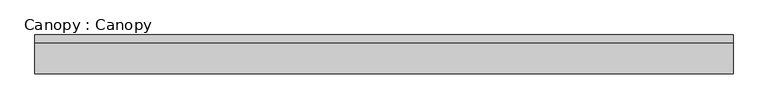
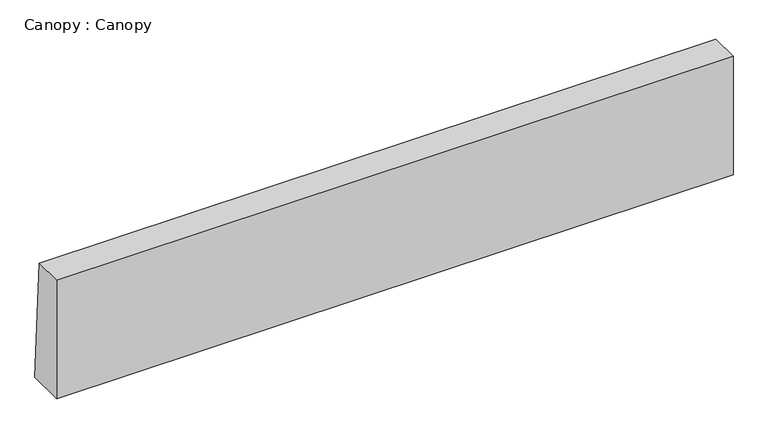
"""IFC4 building model written with IfcOpenShell, lengths in millimetres: proxy geometry, Canopy : Canopy."""

import ifcopenshell
import ifcopenshell.guid

model = None  # the IFC model being written
_history = None  # IfcOwnerHistory: only IFC2X3 demands one
_inside = {}  # id of a spatial element -> (the spatial element, [elements in it])
_under = {}  # id of a project, library or spatial element -> (it, [spatial elements below it])
_declared = {}  # id of a project -> (the project, [libraries it declares])
_typed = {}  # id of a type object -> (the type object, [elements of that type])
_made_of = {}  # id of a material, layer set ... -> (it, [elements and type objects made of it])


def new_model(schema):
    """Start an empty IFC model of exactly this schema.

    Asked for "IFC4X3", IfcOpenShell would pick the latest addendum, in which some entities
    have other attributes; the version numbers below select the first issue.
    IFC2X3 requires an IfcOwnerHistory on every rooted entity: one is made here for all.
    """
    global model, _history
    if schema == "IFC4X3":
        model = ifcopenshell.file(schema_version=(4, 3, 0, 0))
    else:
        model = ifcopenshell.file(schema=schema)
    _inside.clear()
    _under.clear()
    _declared.clear()
    _typed.clear()
    _made_of.clear()
    _history = None
    if model.schema == "IFC2X3":
        org = make("IfcOrganization", Name="unknown")
        user = make(
            "IfcPersonAndOrganization",
            ThePerson=make("IfcPerson", FamilyName="unknown"),
            TheOrganization=org,
        )
        app = make(
            "IfcApplication",
            ApplicationDeveloper=org,
            Version="unknown",
            ApplicationFullName="unknown",
            ApplicationIdentifier="unknown",
        )
        _history = make(
            "IfcOwnerHistory",
            OwningUser=user,
            OwningApplication=app,
            ChangeAction="ADDED",
            CreationDate=0,
        )
    return model


def make(cls, **values):
    """One entity of the class cls with the attributes given. An attribute that is None is left unset."""
    return model.create_entity(
        cls, **{name: value for name, value in values.items() if value is not None}
    )


def rooted(cls, **values):
    """An entity with a GlobalId (a new one), such as an element, a storey or a relation."""
    return make(cls, GlobalId=ifcopenshell.guid.new(), OwnerHistory=_history, **values)


def si_unit(unit_type, name, prefix=None):
    """IfcSIUnit, for example si_unit("LENGTHUNIT", "METRE", prefix="MILLI")."""
    return make("IfcSIUnit", UnitType=unit_type, Prefix=prefix, Name=name)


def assignment(units):
    """IfcUnitAssignment: the units of a project."""
    return None if units is None else make("IfcUnitAssignment", Units=units)


def point(xyz):
    """IfcCartesianPoint."""
    return None if xyz is None else make("IfcCartesianPoint", Coordinates=xyz)


def direction(xyz):
    """IfcDirection."""
    return None if xyz is None else make("IfcDirection", DirectionRatios=xyz)


def frame(location, z_axis=None, x_axis=None):
    """IfcAxis2Placement3D, a coordinate frame: its origin and axes. An axis left out is left unset."""
    return make(
        "IfcAxis2Placement3D",
        Location=point(location),
        Axis=direction(z_axis),
        RefDirection=direction(x_axis),
    )


def origin():
    """The frame at (0, 0, 0) with its axes left unset."""
    return frame((0.0, 0.0, 0.0))


def place(relative_to, where):
    """IfcLocalPlacement: puts the frame where relative to a parent placement (None: the world)."""
    return make(
        "IfcLocalPlacement", PlacementRelTo=relative_to, RelativePlacement=where
    )


def context(
    kind, dimensions, precision=None, world=None, true_north=None, identifier=None
):
    """IfcGeometricRepresentationContext, for example the 3D "Model" context."""
    return make(
        "IfcGeometricRepresentationContext",
        ContextIdentifier=identifier,
        ContextType=kind,
        CoordinateSpaceDimension=dimensions,
        Precision=precision,
        WorldCoordinateSystem=world,
        TrueNorth=true_north,
    )


def project(units=None, contexts=None):
    """IfcProject with its units and contexts."""
    return rooted(
        "IfcProject",
        Name="project",
        RepresentationContexts=contexts,
        UnitsInContext=assignment(units),
    )


def spatial(cls, under=None, at=None, **own):
    """A site, building, storey or space (cls), placed at a placement, below another one or the project."""
    s = rooted(cls, ObjectPlacement=at, **own)
    if under is not None:
        _under.setdefault(under.id(), (under, []))[1].append(s)
    return s


def polyline(points):
    """IfcPolyline through the points."""
    return make("IfcPolyline", Points=[point(p) for p in points])


def outline(outer, holes=None, kind="AREA"):
    """IfcArbitraryClosedProfileDef: a profile drawn as a closed curve; with holes, ...WithVoids."""
    if holes is None:
        return make("IfcArbitraryClosedProfileDef", ProfileType=kind, OuterCurve=outer)
    return make(
        "IfcArbitraryProfileDefWithVoids",
        ProfileType=kind,
        OuterCurve=outer,
        InnerCurves=holes,
    )


def extrude(swept, where, along, depth):
    """IfcExtrudedAreaSolid: the profile swept, set in the frame where, extruded along a direction by depth."""
    return make(
        "IfcExtrudedAreaSolid",
        SweptArea=swept,
        Position=where,
        ExtrudedDirection=direction(along),
        Depth=depth,
    )


def shape(context_of_items, identifier, shape_type, items):
    """IfcShapeRepresentation: the items that make up one representation, for example the "Body"."""
    return make(
        "IfcShapeRepresentation",
        ContextOfItems=context_of_items,
        RepresentationIdentifier=identifier,
        RepresentationType=shape_type,
        Items=items,
    )


def source(mapping_origin, context_of_items, identifier, shape_type, items):
    """IfcRepresentationMap: a shape defined once, which mapped items show again and again."""
    return make(
        "IfcRepresentationMap",
        MappingOrigin=mapping_origin,
        MappedRepresentation=shape(context_of_items, identifier, shape_type, items),
    )


def transform(
    local_origin,
    x_axis=None,
    y_axis=None,
    z_axis=None,
    scale=None,
    scale2=None,
    scale3=None,
    uniform=True,
):
    """IfcCartesianTransformationOperator3D, or its non-uniform kind. x_axis, y_axis, z_axis: its Axis1, 2, 3."""
    if uniform:
        return make(
            "IfcCartesianTransformationOperator3D",
            Axis1=direction(x_axis),
            Axis2=direction(y_axis),
            LocalOrigin=point(local_origin),
            Scale=scale,
            Axis3=direction(z_axis),
        )
    return make(
        "IfcCartesianTransformationOperator3DnonUniform",
        Axis1=direction(x_axis),
        Axis2=direction(y_axis),
        LocalOrigin=point(local_origin),
        Scale=scale,
        Axis3=direction(z_axis),
        Scale2=scale2,
        Scale3=scale3,
    )


def mapped(mapping_source, mapping_target):
    """IfcMappedItem: shows the shape of a source again, moved by a transform."""
    return make(
        "IfcMappedItem", MappingSource=mapping_source, MappingTarget=mapping_target
    )


def made_of(thing, what):
    """Note that an element or type object is made of a material, layer set ...; save() writes the relation."""
    if what is not None:
        _made_of.setdefault(what.id(), (what, []))[1].append(thing)
    return thing


def element(
    cls,
    number,
    at=None,
    inside=None,
    cuts=None,
    type_object=None,
    material=None,
    context=None,
    identifier="Body",
    shape_type=None,
    held_by="IfcProductDefinitionShape",
    body=None,
    shapes=None,
    **own,
):
    """One element of the class cls, such as IfcWall. Its Tag is "e" and its number.

    at: its placement. inside: the storey or other place that contains it. cuts: it is an
    opening in that element (IfcRelVoidsElement). A single representation is given by context,
    identifier, shape_type and body (its items); several are given by shapes. held_by: the class
    of the entity that holds the representations. save() writes the other relations.
    """
    e = rooted(cls, Tag="e%d" % number, ObjectPlacement=at, **own)
    if body is not None:
        shapes = [shape(context, identifier, shape_type, body)]
    if shapes is not None:
        e.Representation = make(held_by, Representations=shapes)
    if inside is not None:
        _inside.setdefault(inside.id(), (inside, []))[1].append(e)
    if cuts is not None:
        rooted(
            "IfcRelVoidsElement", RelatingBuildingElement=cuts, RelatedOpeningElement=e
        )
    if type_object is not None:
        _typed.setdefault(type_object.id(), (type_object, []))[1].append(e)
    return made_of(e, material)


def aggregate(whole, parts):
    """IfcRelAggregates: a whole, such as a stair, and the parts it consists of."""
    return rooted("IfcRelAggregates", RelatingObject=whole, RelatedObjects=parts)


def save(model, path):
    """Write the relations noted so far, then the file.

    IfcRelAggregates (storeys below a building ...), IfcRelContainedInSpatialStructure (elements
    in a storey), IfcRelDefinesByType, IfcRelAssociatesMaterial and IfcRelDeclares: one each for
    every whole, place, type object, material and project.
    """
    for whole, parts in _under.values():
        aggregate(whole, parts)
    for where, things in _inside.values():
        rooted(
            "IfcRelContainedInSpatialStructure",
            RelatedElements=things,
            RelatingStructure=where,
        )
    for kind, things in _typed.values():
        rooted("IfcRelDefinesByType", RelatedObjects=things, RelatingType=kind)
    for what, things in _made_of.values():
        rooted("IfcRelAssociatesMaterial", RelatedObjects=things, RelatingMaterial=what)
    for by, libraries in _declared.values():
        rooted("IfcRelDeclares", RelatingContext=by, RelatedDefinitions=libraries)
    model.write(path)


def canopy_canopy_b27b2f1c(model_context):
    return source(origin(), model_context, "Body", "SweptSolid", [
        extrude(outline(polyline([(150.0, 0.0), (0.0, 0.0), (0.0, 500.0), (120.0, 500.0), (150.0, 0.0)])), frame((-1350.0, 0.0, 0.0), z_axis=(1.0, 0.0, 0.0), x_axis=(0.0, 1.0, 0.0)), (0.0, 0.0, 1.0), 2700.0),
    ])


if __name__ == "__main__":
    model = new_model("IFC4")
    model_context = context("Model", 3, world=origin())
    ifc_project = project(units=[si_unit("LENGTHUNIT", "METRE", prefix="MILLI")], contexts=[model_context])
    site = spatial("IfcSite", under=ifc_project)
    building = spatial("IfcBuilding", under=site)
    placement = place(None, origin())
    canopy_canopy_shape = canopy_canopy_b27b2f1c(model_context)
    element("IfcBuildingElementProxy", 1, Name="Canopy : Canopy", ObjectType="Canopy : Canopy", at=placement, inside=building, context=model_context, shape_type="MappedRepresentation", body=[
        mapped(canopy_canopy_shape, transform((0.0, 0.0, 0.0), x_axis=(1.0, 0.0, 0.0), y_axis=(0.0, 1.0, 0.0), z_axis=(0.0, 0.0, 1.0))),
    ])
    save(model, "model.ifc")

# Revit data of these elements
# Type "Canopy : Canopy"
#   Type Comments = "CV-AG"
#   H_Rebar Ratio = 0.1
#   Canopy Width [instance default] = 1700 mm
#   Canopy Length [instance default] = 1000 mm
#   Canopy L.P = 120 mm
#   Canopy H.P = 150 mm
#   구조재료 = Concrete_f'c=28MPa(Cylender)
#   Default Elevation = 0
# Element 1 (IfcBuildingElementProxy, "Canopy : Canopy")
#   Canopy Width = 2700 mm
#   Canopy Length = 500 mm
#   Materials on its faces: "Concrete_f'c=28MPa(Cylender)"
# Materials
#   "Concrete_f'c=28MPa(Cylender)": class "Concrete", colour RGB 176 176 176, transparency 0, Description = "Reinf. Conc.", Cost = 0, Image = Concrete.Cast-In-Place.Flat.Polished.Grey.jpg
